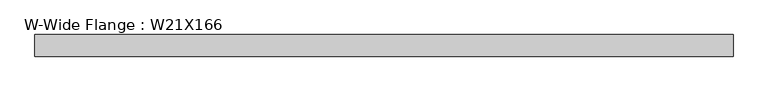
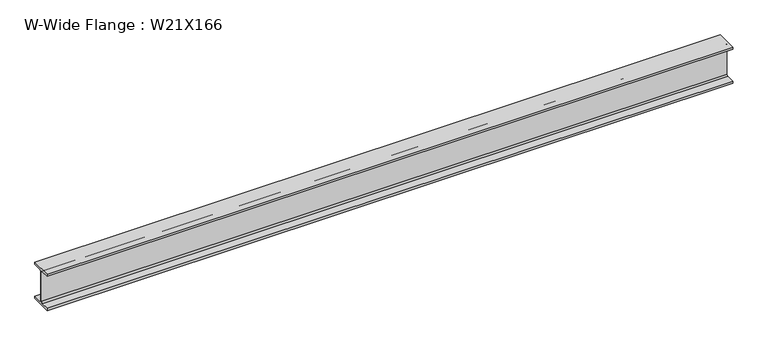
"""IFC4 building model written with IfcOpenShell, lengths in millimetres: beam geometry, W-Wide Flange : W21X166."""

from ifc_helpers import new_model, si_unit, point, frame, frame_2d, origin, place, context, project, spatial, polyline, circle_curve, trimmed, segment, composite_curve, outline, extrude, source, transform, mapped, element, save


def w_wide_flange_w21x166_82cd9a53(model_context):
    return source(origin(), model_context, "Body", "SweptSolid", [
        extrude(outline(composite_curve([segment(polyline([(157.48, -251.206), (157.48, -285.75), (-157.48, -285.75), (-157.48, -251.206), (-32.131, -251.206)]), True, "CONTINUOUS"), segment(trimmed(circle_curve(frame_2d((-32.131, -228.6)), 22.606), [point((-32.131, -251.206))], [point((-9.525, -228.6))], True, "CARTESIAN"), True, "CONTINUOUS"), segment(polyline([(-9.525, -228.6), (-9.525, 228.6)]), True, "CONTINUOUS"), segment(trimmed(circle_curve(frame_2d((-32.131, 228.6)), 22.606), [point((-9.525, 228.6))], [point((-32.131, 251.206))], True, "CARTESIAN"), True, "CONTINUOUS"), segment(polyline([(-32.131, 251.206), (-157.48, 251.206), (-157.48, 285.75), (157.48, 285.75), (157.48, 251.206), (32.131, 251.206)]), True, "CONTINUOUS"), segment(trimmed(circle_curve(frame_2d((32.131, 228.6)), 22.606), [point((32.131, 251.206))], [point((9.525, 228.6))], True, "CARTESIAN"), True, "CONTINUOUS"), segment(polyline([(9.525, 228.6), (9.525, -228.6)]), True, "CONTINUOUS"), segment(trimmed(circle_curve(frame_2d((32.131, -228.6)), 22.606), [point((9.525, -228.6))], [point((32.131, -251.206))], True, "CARTESIAN"), True, "CONTINUOUS"), segment(polyline([(32.131, -251.206), (157.48, -251.206)]), True, "CONTINUOUS")], self_intersect=False)), frame((-5180.0235462, 0.0, 0.0), z_axis=(1.0, 0.0, 0.0), x_axis=(0.0, 1.0, 0.0)), (0.0, 0.0, 1.0), 10182.9648149),
    ])


if __name__ == "__main__":
    model = new_model("IFC4")
    model_context = context("Model", 3, world=origin())
    ifc_project = project(units=[si_unit("LENGTHUNIT", "METRE", prefix="MILLI")], contexts=[model_context])
    site = spatial("IfcSite", under=ifc_project)
    building = spatial("IfcBuilding", under=site)
    placement = place(None, origin())
    w_wide_flange_w21x166_shape = w_wide_flange_w21x166_82cd9a53(model_context)
    element("IfcBeam", 1, ObjectType="W-Wide Flange : W21X166", at=placement, inside=building, context=model_context, shape_type="MappedRepresentation", body=[
        mapped(w_wide_flange_w21x166_shape, transform((0.0, 0.0, 0.0), x_axis=(1.0, 0.0, 0.0), y_axis=(0.0, 1.0, 0.0), z_axis=(0.0, 0.0, 1.0))),
    ])
    save(model, "model.ifc")

# Revit data of these elements
# Type "W-Wide Flange : W21X166"
#   Assembly Code = "B10"
#   W = 166
#   Length [instance default] = 5' - 0"
#   bf = 1' - 0.4"
#   d = 1' - 10 1/2"
#   k = 0' - 2 1/4"
#   k2 = 0' - 0.89"
#   tf = 0' - 1.36"
#   tw = 0' - 0 3/4"
#   A = 0.338889 SF
#   Structural Material [instance default] = Steel ASTM A992
# Element 1 (IfcBeam, "W-Wide Flange : W21X166")
#   Structural Material = Steel
#   Materials on its faces: "Steel"
# Materials
#   "Steel ASTM A992": class "Metal", colour RGB 199 199 199, transparency 0, Description = "Structural steel 50ksi", Cost = 0
#   "Steel": class "Metal", colour RGB 118 118 114, transparency 0, Description = "Steel, mill finish", Cost = 0
